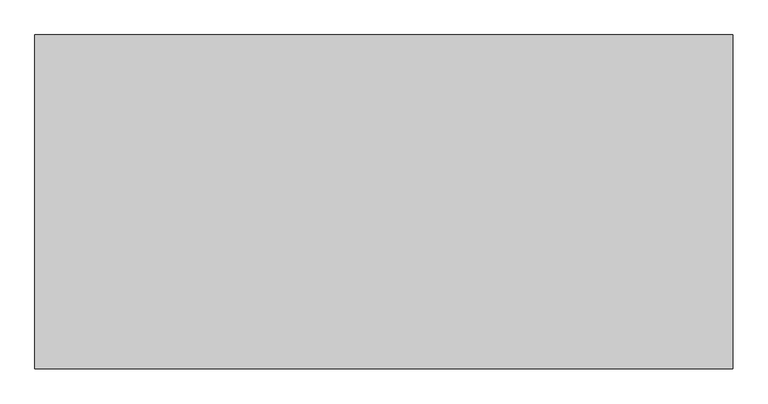
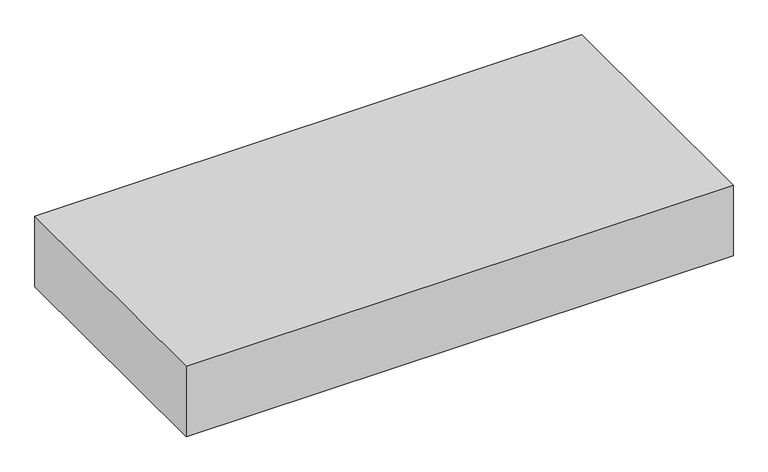
"""IFC4 building model written with IfcOpenShell, lengths in millimetres: proxy geometry, Space Planning Box_hec : Space Planning Box_hec."""

import ifcopenshell
import ifcopenshell.guid

model = None  # the IFC model being written
_history = None  # IfcOwnerHistory: only IFC2X3 demands one
_inside = {}  # id of a spatial element -> (the spatial element, [elements in it])
_under = {}  # id of a project, library or spatial element -> (it, [spatial elements below it])
_declared = {}  # id of a project -> (the project, [libraries it declares])
_typed = {}  # id of a type object -> (the type object, [elements of that type])
_made_of = {}  # id of a material, layer set ... -> (it, [elements and type objects made of it])


def new_model(schema):
    """Start an empty IFC model of exactly this schema.

    Asked for "IFC4X3", IfcOpenShell would pick the latest addendum, in which some entities
    have other attributes; the version numbers below select the first issue.
    IFC2X3 requires an IfcOwnerHistory on every rooted entity: one is made here for all.
    """
    global model, _history
    if schema == "IFC4X3":
        model = ifcopenshell.file(schema_version=(4, 3, 0, 0))
    else:
        model = ifcopenshell.file(schema=schema)
    _inside.clear()
    _under.clear()
    _declared.clear()
    _typed.clear()
    _made_of.clear()
    _history = None
    if model.schema == "IFC2X3":
        org = make("IfcOrganization", Name="unknown")
        user = make(
            "IfcPersonAndOrganization",
            ThePerson=make("IfcPerson", FamilyName="unknown"),
            TheOrganization=org,
        )
        app = make(
            "IfcApplication",
            ApplicationDeveloper=org,
            Version="unknown",
            ApplicationFullName="unknown",
            ApplicationIdentifier="unknown",
        )
        _history = make(
            "IfcOwnerHistory",
            OwningUser=user,
            OwningApplication=app,
            ChangeAction="ADDED",
            CreationDate=0,
        )
    return model


def make(cls, **values):
    """One entity of the class cls with the attributes given. An attribute that is None is left unset."""
    return model.create_entity(
        cls, **{name: value for name, value in values.items() if value is not None}
    )


def rooted(cls, **values):
    """An entity with a GlobalId (a new one), such as an element, a storey or a relation."""
    return make(cls, GlobalId=ifcopenshell.guid.new(), OwnerHistory=_history, **values)


def si_unit(unit_type, name, prefix=None):
    """IfcSIUnit, for example si_unit("LENGTHUNIT", "METRE", prefix="MILLI")."""
    return make("IfcSIUnit", UnitType=unit_type, Prefix=prefix, Name=name)


def assignment(units):
    """IfcUnitAssignment: the units of a project."""
    return None if units is None else make("IfcUnitAssignment", Units=units)


def point(xyz):
    """IfcCartesianPoint."""
    return None if xyz is None else make("IfcCartesianPoint", Coordinates=xyz)


def direction(xyz):
    """IfcDirection."""
    return None if xyz is None else make("IfcDirection", DirectionRatios=xyz)


def frame(location, z_axis=None, x_axis=None):
    """IfcAxis2Placement3D, a coordinate frame: its origin and axes. An axis left out is left unset."""
    return make(
        "IfcAxis2Placement3D",
        Location=point(location),
        Axis=direction(z_axis),
        RefDirection=direction(x_axis),
    )


def origin():
    """The frame at (0, 0, 0) with its axes left unset."""
    return frame((0.0, 0.0, 0.0))


def origin_with_axes():
    """The frame at (0, 0, 0) with the z axis (0, 0, 1) and the x axis (1, 0, 0) written out."""
    return frame((0.0, 0.0, 0.0), z_axis=(0.0, 0.0, 1.0), x_axis=(1.0, 0.0, 0.0))


def place(relative_to, where):
    """IfcLocalPlacement: puts the frame where relative to a parent placement (None: the world)."""
    return make(
        "IfcLocalPlacement", PlacementRelTo=relative_to, RelativePlacement=where
    )


def context(
    kind, dimensions, precision=None, world=None, true_north=None, identifier=None
):
    """IfcGeometricRepresentationContext, for example the 3D "Model" context."""
    return make(
        "IfcGeometricRepresentationContext",
        ContextIdentifier=identifier,
        ContextType=kind,
        CoordinateSpaceDimension=dimensions,
        Precision=precision,
        WorldCoordinateSystem=world,
        TrueNorth=true_north,
    )


def project(units=None, contexts=None):
    """IfcProject with its units and contexts."""
    return rooted(
        "IfcProject",
        Name="project",
        RepresentationContexts=contexts,
        UnitsInContext=assignment(units),
    )


def spatial(cls, under=None, at=None, **own):
    """A site, building, storey or space (cls), placed at a placement, below another one or the project."""
    s = rooted(cls, ObjectPlacement=at, **own)
    if under is not None:
        _under.setdefault(under.id(), (under, []))[1].append(s)
    return s


def polyline(points):
    """IfcPolyline through the points."""
    return make("IfcPolyline", Points=[point(p) for p in points])


def outline(outer, holes=None, kind="AREA"):
    """IfcArbitraryClosedProfileDef: a profile drawn as a closed curve; with holes, ...WithVoids."""
    if holes is None:
        return make("IfcArbitraryClosedProfileDef", ProfileType=kind, OuterCurve=outer)
    return make(
        "IfcArbitraryProfileDefWithVoids",
        ProfileType=kind,
        OuterCurve=outer,
        InnerCurves=holes,
    )


def extrude(swept, where, along, depth):
    """IfcExtrudedAreaSolid: the profile swept, set in the frame where, extruded along a direction by depth."""
    return make(
        "IfcExtrudedAreaSolid",
        SweptArea=swept,
        Position=where,
        ExtrudedDirection=direction(along),
        Depth=depth,
    )


def shape(context_of_items, identifier, shape_type, items):
    """IfcShapeRepresentation: the items that make up one representation, for example the "Body"."""
    return make(
        "IfcShapeRepresentation",
        ContextOfItems=context_of_items,
        RepresentationIdentifier=identifier,
        RepresentationType=shape_type,
        Items=items,
    )


def source(mapping_origin, context_of_items, identifier, shape_type, items):
    """IfcRepresentationMap: a shape defined once, which mapped items show again and again."""
    return make(
        "IfcRepresentationMap",
        MappingOrigin=mapping_origin,
        MappedRepresentation=shape(context_of_items, identifier, shape_type, items),
    )


def transform(
    local_origin,
    x_axis=None,
    y_axis=None,
    z_axis=None,
    scale=None,
    scale2=None,
    scale3=None,
    uniform=True,
):
    """IfcCartesianTransformationOperator3D, or its non-uniform kind. x_axis, y_axis, z_axis: its Axis1, 2, 3."""
    if uniform:
        return make(
            "IfcCartesianTransformationOperator3D",
            Axis1=direction(x_axis),
            Axis2=direction(y_axis),
            LocalOrigin=point(local_origin),
            Scale=scale,
            Axis3=direction(z_axis),
        )
    return make(
        "IfcCartesianTransformationOperator3DnonUniform",
        Axis1=direction(x_axis),
        Axis2=direction(y_axis),
        LocalOrigin=point(local_origin),
        Scale=scale,
        Axis3=direction(z_axis),
        Scale2=scale2,
        Scale3=scale3,
    )


def mapped(mapping_source, mapping_target):
    """IfcMappedItem: shows the shape of a source again, moved by a transform."""
    return make(
        "IfcMappedItem", MappingSource=mapping_source, MappingTarget=mapping_target
    )


def made_of(thing, what):
    """Note that an element or type object is made of a material, layer set ...; save() writes the relation."""
    if what is not None:
        _made_of.setdefault(what.id(), (what, []))[1].append(thing)
    return thing


def element(
    cls,
    number,
    at=None,
    inside=None,
    cuts=None,
    type_object=None,
    material=None,
    context=None,
    identifier="Body",
    shape_type=None,
    held_by="IfcProductDefinitionShape",
    body=None,
    shapes=None,
    **own,
):
    """One element of the class cls, such as IfcWall. Its Tag is "e" and its number.

    at: its placement. inside: the storey or other place that contains it. cuts: it is an
    opening in that element (IfcRelVoidsElement). A single representation is given by context,
    identifier, shape_type and body (its items); several are given by shapes. held_by: the class
    of the entity that holds the representations. save() writes the other relations.
    """
    e = rooted(cls, Tag="e%d" % number, ObjectPlacement=at, **own)
    if body is not None:
        shapes = [shape(context, identifier, shape_type, body)]
    if shapes is not None:
        e.Representation = make(held_by, Representations=shapes)
    if inside is not None:
        _inside.setdefault(inside.id(), (inside, []))[1].append(e)
    if cuts is not None:
        rooted(
            "IfcRelVoidsElement", RelatingBuildingElement=cuts, RelatedOpeningElement=e
        )
    if type_object is not None:
        _typed.setdefault(type_object.id(), (type_object, []))[1].append(e)
    return made_of(e, material)


def aggregate(whole, parts):
    """IfcRelAggregates: a whole, such as a stair, and the parts it consists of."""
    return rooted("IfcRelAggregates", RelatingObject=whole, RelatedObjects=parts)


def save(model, path):
    """Write the relations noted so far, then the file.

    IfcRelAggregates (storeys below a building ...), IfcRelContainedInSpatialStructure (elements
    in a storey), IfcRelDefinesByType, IfcRelAssociatesMaterial and IfcRelDeclares: one each for
    every whole, place, type object, material and project.
    """
    for whole, parts in _under.values():
        aggregate(whole, parts)
    for where, things in _inside.values():
        rooted(
            "IfcRelContainedInSpatialStructure",
            RelatedElements=things,
            RelatingStructure=where,
        )
    for kind, things in _typed.values():
        rooted("IfcRelDefinesByType", RelatedObjects=things, RelatingType=kind)
    for what, things in _made_of.values():
        rooted("IfcRelAssociatesMaterial", RelatedObjects=things, RelatingMaterial=what)
    for by, libraries in _declared.values():
        rooted("IfcRelDeclares", RelatingContext=by, RelatedDefinitions=libraries)
    model.write(path)


def generic_models_b3b0fa1d(model_context):
    return source(origin(), model_context, "Body", "SweptSolid", [
        extrude(outline(polyline([(21950.0, 10500.0), (21950.0, -10500.0), (-21950.0, -10500.0), (-21950.0, 10500.0), (21950.0, 10500.0)])), origin_with_axes(), (0.0, 0.0, 1.0), 6000.0),
    ])


if __name__ == "__main__":
    model = new_model("IFC4")
    model_context = context("Model", 3, world=origin())
    ifc_project = project(units=[si_unit("LENGTHUNIT", "METRE", prefix="MILLI")], contexts=[model_context])
    site = spatial("IfcSite", under=ifc_project)
    building = spatial("IfcBuilding", under=site)
    placement = place(None, origin())
    generic_models_shape = generic_models_b3b0fa1d(model_context)
    element("IfcBuildingElementProxy", 1, Name="Space Planning Box_hec : Space Planning Box_hec", ObjectType="Space Planning Box_hec : Space Planning Box_hec", at=placement, inside=building, context=model_context, shape_type="MappedRepresentation", body=[
        mapped(generic_models_shape, transform((0.0, 0.0, 0.0), x_axis=(1.0, 0.0, 0.0), y_axis=(0.0, 1.0, 0.0), z_axis=(0.0, 0.0, 1.0))),
    ])
    save(model, "model.ifc")

# Revit data of these elements
# Type "Space Planning Box_hec : Space Planning Box_hec"
#   Type Comments = "..."
#   Room Name [instance default] = "?"
#   Interior Finish [instance default] = ""
#   Exterior Finish [instance default] = ""
#   Department [instance default] = ""
#   Assembly Code = "..."
#   Width [instance default] = 1524 mm
#   Program Area [instance default] = 0 m²
#   Length [instance default] = 1524 mm
#   Height [instance default] = 1524 mm
#   Area [instance default] = 2.32258 m²
#   Fill Color [instance default] = Cyan
#   Default Elevation = 0
# Element 1 (IfcBuildingElementProxy, "Space Planning Box_hec : Space Planning Box_hec")
#   Room Name = "Corridor"
#   Interior Finish = "IF2-1"
#   Exterior Finish = "EF1"
#   Department = "AR"
#   Width = 43900 mm
#   Length = 21000 mm
#   Height = 6000 mm
#   Area = 921.9 m²
#   Fill Color = Lavender
#   Materials on its faces: "Lavender"
# Materials
#   "Cyan": class "Generic", colour RGB 0 255 255, transparency 0.2, Cost = 0
#   "Lavender": class "Generic", colour RGB 186 85 211, transparency 0.2, Cost = 0
